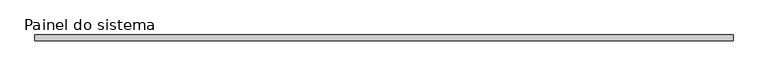
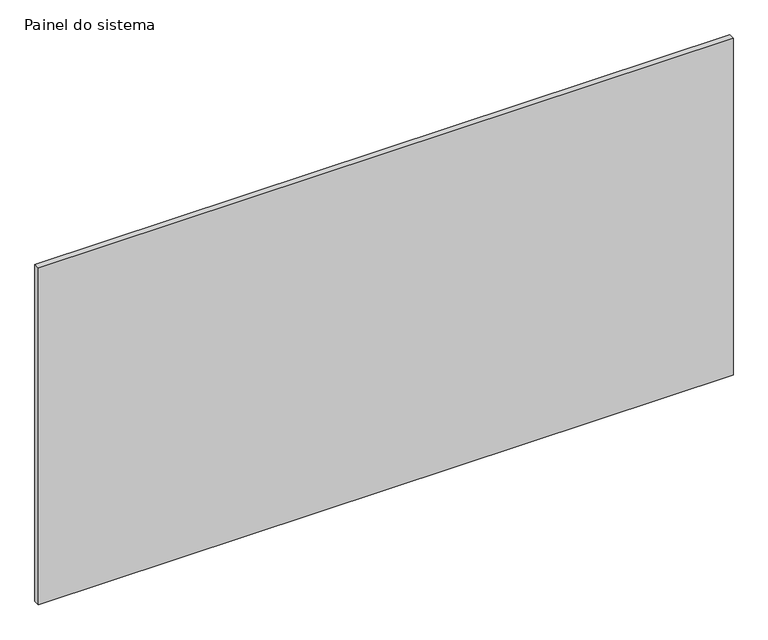
"""IFC4 building model written with IfcOpenShell, lengths in millimetres: plate geometry, Painel do sistema : Envidraçado."""

from ifc_helpers import new_model, si_unit, origin, origin_with_axes, place, context, project, spatial, polyline, outline, extrude, source, transform, mapped, element, save


def painel_do_sistema_619734db(model_context):
    return source(origin(), model_context, "Body", "SweptSolid", [
        extrude(outline(polyline([(1462.5000305, -49.5), (-1462.5000305, -49.5), (-1462.5000305, -24.5), (1462.5000305, -24.5), (1462.5000305, -49.5)])), origin_with_axes(), (0.0, 0.0, 1.0), 1500.0),
    ])


if __name__ == "__main__":
    model = new_model("IFC4")
    model_context = context("Model", 3, world=origin())
    ifc_project = project(units=[si_unit("LENGTHUNIT", "METRE", prefix="MILLI")], contexts=[model_context])
    site = spatial("IfcSite", under=ifc_project)
    building = spatial("IfcBuilding", under=site)
    placement = place(None, origin())
    painel_do_sistema_shape = painel_do_sistema_619734db(model_context)
    element("IfcPlate", 1, ObjectType="Painel do sistema : Envidraçado", at=placement, inside=building, context=model_context, shape_type="MappedRepresentation", body=[
        mapped(painel_do_sistema_shape, transform((0.0, 0.0, 0.0), x_axis=(1.0, 0.0, 0.0), y_axis=(0.0, 1.0, 0.0), z_axis=(0.0, 0.0, 1.0))),
    ])
    save(model, "model.ifc")

# Revit data of these elements
# Type "Painel do sistema : Envidraçado"
#   Construction Type Id = "GSP4R"
#   Analytic Construction = "Vidraça única Pilkington 1/8 pol"
#   Visual Light Transmittance = 0.9
#   Solar Heat Gain Coefficient = 0.86
#   Heat Transfer Coefficient (U) = 6.7069 W/(m²·K)
# Element 1 (IfcPlate, "Painel do sistema : Envidraçado")
#   Materials on its faces: "Vidro"
# Materials
#   "Vidro": class "Vidro", colour RGB 0 128 192, transparency 0.9, Description = "Vidro de sílica", Cost = 0
